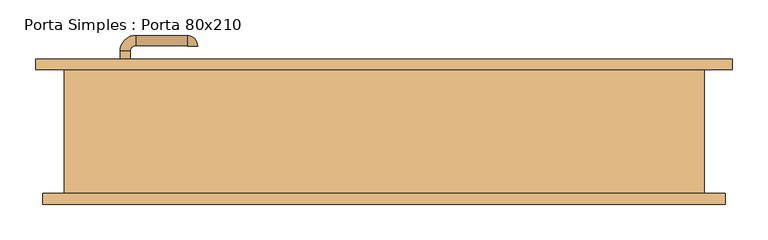
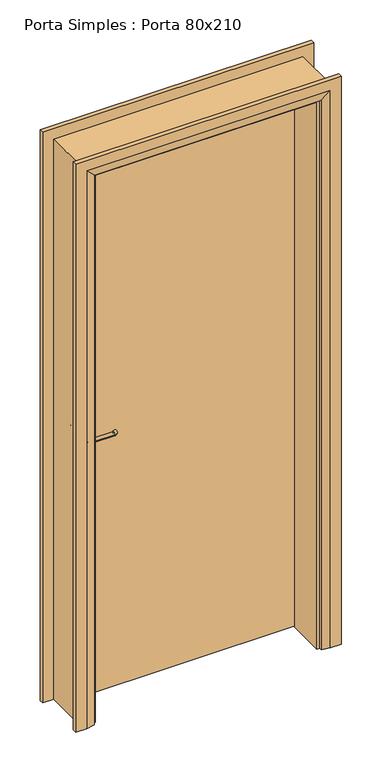
"""IFC4 building model written with IfcOpenShell, lengths in millimetres: door geometry, Porta Simples : Porta 80x210."""

import ifcopenshell
import ifcopenshell.guid

model = None  # the IFC model being written
_history = None  # IfcOwnerHistory: only IFC2X3 demands one
_inside = {}  # id of a spatial element -> (the spatial element, [elements in it])
_under = {}  # id of a project, library or spatial element -> (it, [spatial elements below it])
_declared = {}  # id of a project -> (the project, [libraries it declares])
_typed = {}  # id of a type object -> (the type object, [elements of that type])
_made_of = {}  # id of a material, layer set ... -> (it, [elements and type objects made of it])


def new_model(schema):
    """Start an empty IFC model of exactly this schema.

    Asked for "IFC4X3", IfcOpenShell would pick the latest addendum, in which some entities
    have other attributes; the version numbers below select the first issue.
    IFC2X3 requires an IfcOwnerHistory on every rooted entity: one is made here for all.
    """
    global model, _history
    if schema == "IFC4X3":
        model = ifcopenshell.file(schema_version=(4, 3, 0, 0))
    else:
        model = ifcopenshell.file(schema=schema)
    _inside.clear()
    _under.clear()
    _declared.clear()
    _typed.clear()
    _made_of.clear()
    _history = None
    if model.schema == "IFC2X3":
        org = make("IfcOrganization", Name="unknown")
        user = make(
            "IfcPersonAndOrganization",
            ThePerson=make("IfcPerson", FamilyName="unknown"),
            TheOrganization=org,
        )
        app = make(
            "IfcApplication",
            ApplicationDeveloper=org,
            Version="unknown",
            ApplicationFullName="unknown",
            ApplicationIdentifier="unknown",
        )
        _history = make(
            "IfcOwnerHistory",
            OwningUser=user,
            OwningApplication=app,
            ChangeAction="ADDED",
            CreationDate=0,
        )
    return model


def make(cls, **values):
    """One entity of the class cls with the attributes given. An attribute that is None is left unset."""
    return model.create_entity(
        cls, **{name: value for name, value in values.items() if value is not None}
    )


def rooted(cls, **values):
    """An entity with a GlobalId (a new one), such as an element, a storey or a relation."""
    return make(cls, GlobalId=ifcopenshell.guid.new(), OwnerHistory=_history, **values)


def si_unit(unit_type, name, prefix=None):
    """IfcSIUnit, for example si_unit("LENGTHUNIT", "METRE", prefix="MILLI")."""
    return make("IfcSIUnit", UnitType=unit_type, Prefix=prefix, Name=name)


def assignment(units):
    """IfcUnitAssignment: the units of a project."""
    return None if units is None else make("IfcUnitAssignment", Units=units)


def point(xyz):
    """IfcCartesianPoint."""
    return None if xyz is None else make("IfcCartesianPoint", Coordinates=xyz)


def direction(xyz):
    """IfcDirection."""
    return None if xyz is None else make("IfcDirection", DirectionRatios=xyz)


def frame(location, z_axis=None, x_axis=None):
    """IfcAxis2Placement3D, a coordinate frame: its origin and axes. An axis left out is left unset."""
    return make(
        "IfcAxis2Placement3D",
        Location=point(location),
        Axis=direction(z_axis),
        RefDirection=direction(x_axis),
    )


def frame_2d(location, x_axis=None):
    """IfcAxis2Placement2D, a coordinate frame in the plane: its origin and x axis."""
    return make(
        "IfcAxis2Placement2D", Location=point(location), RefDirection=direction(x_axis)
    )


def origin():
    """The frame at (0, 0, 0) with its axes left unset."""
    return frame((0.0, 0.0, 0.0))


def place(relative_to, where):
    """IfcLocalPlacement: puts the frame where relative to a parent placement (None: the world)."""
    return make(
        "IfcLocalPlacement", PlacementRelTo=relative_to, RelativePlacement=where
    )


def context(
    kind, dimensions, precision=None, world=None, true_north=None, identifier=None
):
    """IfcGeometricRepresentationContext, for example the 3D "Model" context."""
    return make(
        "IfcGeometricRepresentationContext",
        ContextIdentifier=identifier,
        ContextType=kind,
        CoordinateSpaceDimension=dimensions,
        Precision=precision,
        WorldCoordinateSystem=world,
        TrueNorth=true_north,
    )


def project(units=None, contexts=None):
    """IfcProject with its units and contexts."""
    return rooted(
        "IfcProject",
        Name="project",
        RepresentationContexts=contexts,
        UnitsInContext=assignment(units),
    )


def spatial(cls, under=None, at=None, **own):
    """A site, building, storey or space (cls), placed at a placement, below another one or the project."""
    s = rooted(cls, ObjectPlacement=at, **own)
    if under is not None:
        _under.setdefault(under.id(), (under, []))[1].append(s)
    return s


def polyline(points):
    """IfcPolyline through the points."""
    return make("IfcPolyline", Points=[point(p) for p in points])


def circle_curve(where, radius):
    """IfcCircle in the frame where."""
    return make("IfcCircle", Position=where, Radius=radius)


def ellipse_curve(where, semi_axis1, semi_axis2):
    """IfcEllipse in the frame where."""
    return make(
        "IfcEllipse", Position=where, SemiAxis1=semi_axis1, SemiAxis2=semi_axis2
    )


def trimmed(basis, trim1, trim2, sense, master):
    """IfcTrimmedCurve: the piece of a basis curve between two trims."""
    return make(
        "IfcTrimmedCurve",
        BasisCurve=basis,
        Trim1=trim1,
        Trim2=trim2,
        SenseAgreement=sense,
        MasterRepresentation=master,
    )


def segment(curve, same_sense, transition):
    """IfcCompositeCurveSegment."""
    return make(
        "IfcCompositeCurveSegment",
        Transition=transition,
        SameSense=same_sense,
        ParentCurve=curve,
    )


def composite_curve(segments, self_intersect=None):
    """IfcCompositeCurve: segments joined end to end."""
    return make("IfcCompositeCurve", Segments=segments, SelfIntersect=self_intersect)


def outline(outer, holes=None, kind="AREA"):
    """IfcArbitraryClosedProfileDef: a profile drawn as a closed curve; with holes, ...WithVoids."""
    if holes is None:
        return make("IfcArbitraryClosedProfileDef", ProfileType=kind, OuterCurve=outer)
    return make(
        "IfcArbitraryProfileDefWithVoids",
        ProfileType=kind,
        OuterCurve=outer,
        InnerCurves=holes,
    )


def extrude(swept, where, along, depth):
    """IfcExtrudedAreaSolid: the profile swept, set in the frame where, extruded along a direction by depth."""
    return make(
        "IfcExtrudedAreaSolid",
        SweptArea=swept,
        Position=where,
        ExtrudedDirection=direction(along),
        Depth=depth,
    )


def faces_of(points, faces, orient=None, outer=None):
    """IfcFace entities. A face is a list of loops; a loop is a list of indices into points, from 0.

    orient and outer hold one flag for each loop. By default every Orientation is true, the
    first loop of a face is its IfcFaceOuterBound and the others are IfcFaceBound.
    """
    made = []
    for i, loops in enumerate(faces):
        bounds = []
        for j, loop in enumerate(loops):
            is_outer = j == 0 if outer is None else outer[i][j]
            bounds.append(
                make(
                    "IfcFaceOuterBound" if is_outer else "IfcFaceBound",
                    Bound=make("IfcPolyLoop", Polygon=[points[k] for k in loop]),
                    Orientation=True if orient is None else orient[i][j],
                )
            )
        made.append(make("IfcFace", Bounds=bounds))
    return made


def faceted_brep(points, faces, orient=None, outer=None, voids=None):
    """IfcFacetedBrep: a solid bounded by flat faces; with voids (closed shells), ...WithVoids."""
    shared = [point(p) for p in points]
    hull = make("IfcClosedShell", CfsFaces=faces_of(shared, faces, orient, outer))
    if voids is None:
        return make("IfcFacetedBrep", Outer=hull)
    return make(
        "IfcFacetedBrepWithVoids",
        Outer=hull,
        Voids=[
            make(cls, CfsFaces=faces_of(shared, fs, o, b)) for cls, fs, o, b in voids
        ],
    )


def shape(context_of_items, identifier, shape_type, items):
    """IfcShapeRepresentation: the items that make up one representation, for example the "Body"."""
    return make(
        "IfcShapeRepresentation",
        ContextOfItems=context_of_items,
        RepresentationIdentifier=identifier,
        RepresentationType=shape_type,
        Items=items,
    )


def source(mapping_origin, context_of_items, identifier, shape_type, items):
    """IfcRepresentationMap: a shape defined once, which mapped items show again and again."""
    return make(
        "IfcRepresentationMap",
        MappingOrigin=mapping_origin,
        MappedRepresentation=shape(context_of_items, identifier, shape_type, items),
    )


def transform(
    local_origin,
    x_axis=None,
    y_axis=None,
    z_axis=None,
    scale=None,
    scale2=None,
    scale3=None,
    uniform=True,
):
    """IfcCartesianTransformationOperator3D, or its non-uniform kind. x_axis, y_axis, z_axis: its Axis1, 2, 3."""
    if uniform:
        return make(
            "IfcCartesianTransformationOperator3D",
            Axis1=direction(x_axis),
            Axis2=direction(y_axis),
            LocalOrigin=point(local_origin),
            Scale=scale,
            Axis3=direction(z_axis),
        )
    return make(
        "IfcCartesianTransformationOperator3DnonUniform",
        Axis1=direction(x_axis),
        Axis2=direction(y_axis),
        LocalOrigin=point(local_origin),
        Scale=scale,
        Axis3=direction(z_axis),
        Scale2=scale2,
        Scale3=scale3,
    )


def mapped(mapping_source, mapping_target):
    """IfcMappedItem: shows the shape of a source again, moved by a transform."""
    return make(
        "IfcMappedItem", MappingSource=mapping_source, MappingTarget=mapping_target
    )


def made_of(thing, what):
    """Note that an element or type object is made of a material, layer set ...; save() writes the relation."""
    if what is not None:
        _made_of.setdefault(what.id(), (what, []))[1].append(thing)
    return thing


def element(
    cls,
    number,
    at=None,
    inside=None,
    cuts=None,
    type_object=None,
    material=None,
    context=None,
    identifier="Body",
    shape_type=None,
    held_by="IfcProductDefinitionShape",
    body=None,
    shapes=None,
    **own,
):
    """One element of the class cls, such as IfcWall. Its Tag is "e" and its number.

    at: its placement. inside: the storey or other place that contains it. cuts: it is an
    opening in that element (IfcRelVoidsElement). A single representation is given by context,
    identifier, shape_type and body (its items); several are given by shapes. held_by: the class
    of the entity that holds the representations. save() writes the other relations.
    """
    e = rooted(cls, Tag="e%d" % number, ObjectPlacement=at, **own)
    if body is not None:
        shapes = [shape(context, identifier, shape_type, body)]
    if shapes is not None:
        e.Representation = make(held_by, Representations=shapes)
    if inside is not None:
        _inside.setdefault(inside.id(), (inside, []))[1].append(e)
    if cuts is not None:
        rooted(
            "IfcRelVoidsElement", RelatingBuildingElement=cuts, RelatedOpeningElement=e
        )
    if type_object is not None:
        _typed.setdefault(type_object.id(), (type_object, []))[1].append(e)
    return made_of(e, material)


def aggregate(whole, parts):
    """IfcRelAggregates: a whole, such as a stair, and the parts it consists of."""
    return rooted("IfcRelAggregates", RelatingObject=whole, RelatedObjects=parts)


def save(model, path):
    """Write the relations noted so far, then the file.

    IfcRelAggregates (storeys below a building ...), IfcRelContainedInSpatialStructure (elements
    in a storey), IfcRelDefinesByType, IfcRelAssociatesMaterial and IfcRelDeclares: one each for
    every whole, place, type object, material and project.
    """
    for whole, parts in _under.values():
        aggregate(whole, parts)
    for where, things in _inside.values():
        rooted(
            "IfcRelContainedInSpatialStructure",
            RelatedElements=things,
            RelatingStructure=where,
        )
    for kind, things in _typed.values():
        rooted("IfcRelDefinesByType", RelatedObjects=things, RelatingType=kind)
    for what, things in _made_of.values():
        rooted("IfcRelAssociatesMaterial", RelatedObjects=things, RelatingMaterial=what)
    for by, libraries in _declared.values():
        rooted("IfcRelDeclares", RelatingContext=by, RelatedDefinitions=libraries)
    model.write(path)


def plane_surface(at):
    """IfcPlane: the flat surface through the origin of the frame at, square to its z axis."""
    return make("IfcPlane", Position=at)


def cylinder_surface(at, radius):
    """IfcCylindricalSurface: all points at the distance radius from the z axis of the frame at."""
    return make("IfcCylindricalSurface", Position=at, Radius=radius)


def revolved_surface(curve, axis_point, axis_direction):
    """IfcSurfaceOfRevolution: the curve turned about the line through axis_point along axis_direction."""
    return make(
        "IfcSurfaceOfRevolution",
        SweptCurve=make("IfcArbitraryOpenProfileDef", ProfileType="CURVE", Curve=curve),
        AxisPosition=make("IfcAxis1Placement", Location=point(axis_point), Axis=direction(axis_direction)),
    )


def advanced_brep(points, edges, surfaces, faces):
    """IfcAdvancedBrep: a solid bounded by faces that lie on surfaces and meet in shared edges.

    An edge is (start, end): straight between two places in points (the first is 0);
    or (start, end, curve); or (start, end, curve, False) where it runs against its curve.
    A face is (place in surfaces, loops), or (place, loops, False) where it looks against
    its surface's normal. A loop lists edges by number (the first is 1), with a minus sign
    where the edge is run from its end to its start. The first loop is the outer one.
    """
    corners = [point(p) for p in points]
    vertices = [make("IfcVertexPoint", VertexGeometry=c) for c in corners]
    made = []
    for start, end, *more in edges:
        made.append(
            make(
                "IfcEdgeCurve",
                EdgeStart=vertices[start],
                EdgeEnd=vertices[end],
                EdgeGeometry=more[0] if more else make("IfcPolyline", Points=[corners[start], corners[end]]),
                SameSense=more[1] if len(more) > 1 else True,
            )
        )
    hull = []
    for where, loops, *sense in faces:
        bounds = []
        for j, loop in enumerate(loops):
            ring = [make("IfcOrientedEdge", EdgeElement=made[abs(k) - 1], Orientation=k > 0) for k in loop]
            bounds.append(
                make(
                    "IfcFaceOuterBound" if j == 0 else "IfcFaceBound",
                    Bound=make("IfcEdgeLoop", EdgeList=ring),
                    Orientation=True,
                )
            )
        hull.append(make("IfcAdvancedFace", Bounds=bounds, FaceSurface=surfaces[where], SameSense=sense[0] if sense else True))
    return make("IfcAdvancedBrep", Outer=make("IfcClosedShell", CfsFaces=hull))


def porta_simples_porta_80x210_892b00d0(model_context):
    return source(origin(), model_context, "Body", "SolidModel", [
        extrude(outline(composite_curve([segment(trimmed(circle_curve(frame_2d((1050.0, -364.0)), 20.0), [point((1050.0, -384.0))], [point((1050.0, -344.0))], False, "CARTESIAN"), True, "CONTINUOUS"), segment(trimmed(circle_curve(frame_2d((1050.0, -364.0)), 20.0), [point((1050.0, -344.0))], [point((1050.0, -384.0))], False, "CARTESIAN"), True, "CONTINUOUS")], self_intersect=False)), frame((0.0, 41.7070105, 0.0), z_axis=(0.0, 1.0, 0.0), x_axis=(0.0, 0.0, 1.0)), (0.0, 0.0, 1.0), 4.5929895),
        advanced_brep(
        [(-357.0, 41.7070105, 1050.0), (-371.0, 41.7070105, 1050.0), (-371.0, 26.3, 1050.0), (-357.0, 26.3, 1050.0), (-349.0, 4.3, 1050.0), (-349.0, 18.3, 1050.0), (-277.0, 4.3, 1050.0), (-277.0, 18.3, 1050.0), (-276.0, 19.3, 1050.0), (-262.0, 19.3, 1050.0)],
        [
            (0, 1, circle_curve(frame((-364.0, 41.7070105, 1050.0), z_axis=(0.0, 1.0, 0.0), x_axis=(-1.0, 0.0, 0.0)), 7.0)),
            (1, 0, circle_curve(frame((-364.0, 41.7070105, 1050.0), z_axis=(0.0, 1.0, 0.0), x_axis=(-1.0, 0.0, 0.0)), 7.0)),
            (1, 2),
            (2, 3, circle_curve(frame((-364.0, 26.3, 1050.0), z_axis=(0.0, 1.0, 0.0), x_axis=(-1.0, 0.0, 0.0)), 7.0)),
            (3, 0),
            (3, 2, circle_curve(frame((-364.0, 26.3, 1050.0), z_axis=(0.0, 1.0, 0.0), x_axis=(-1.0, 0.0, 0.0)), 7.0)),
            (4, 5, circle_curve(frame((-349.0, 11.3, 1050.0), z_axis=(-1.0, 0.0, 0.0), x_axis=(0.0, -1.0, 0.0)), 7.0)),
            (5, 3, circle_curve(frame((-349.0, 26.3, 1050.0), z_axis=(0.0, 0.0, -1.0), x_axis=(-1.0, 0.0, 0.0)), 8.0)),
            (2, 4, circle_curve(frame((-349.0, 26.3, 1050.0), z_axis=(0.0, 0.0, 1.0), x_axis=(-1.0, 0.0, 0.0)), 22.0)),
            (5, 4, circle_curve(frame((-349.0, 11.3, 1050.0), z_axis=(-1.0, 0.0, 0.0), x_axis=(0.0, -1.0, 0.0)), 7.0)),
            (4, 6),
            (6, 7, circle_curve(frame((-277.0, 11.3, 1050.0), z_axis=(-1.0, 0.0, 0.0), x_axis=(0.0, -1.0, 0.0)), 7.0)),
            (7, 5),
            (7, 6, circle_curve(frame((-277.0, 11.3, 1050.0), z_axis=(-1.0, 0.0, 0.0), x_axis=(0.0, -1.0, 0.0)), 7.0)),
            (8, 9, circle_curve(frame((-269.0, 19.3, 1050.0), z_axis=(0.0, 1.0, 0.0), x_axis=(1.0, 0.0, 0.0)), 7.0)),
            (9, 8, circle_curve(frame((-269.0, 19.3, 1050.0), z_axis=(0.0, 1.0, 0.0), x_axis=(1.0, 0.0, 0.0)), 7.0)),
            (8, 7, circle_curve(frame((-277.0, 19.3, 1050.0), z_axis=(0.0, 0.0, -1.0), x_axis=(0.0, -1.0, 0.0)), 1.0)),
            (6, 9, circle_curve(frame((-277.0, 19.3, 1050.0), z_axis=(0.0, 0.0, 1.0), x_axis=(0.0, -1.0, 0.0)), 15.0)),
        ],
        [
            plane_surface(frame((-364.0, 41.7070105, 1050.0), z_axis=(0.0, 1.0, 0.0), x_axis=(0.0, 0.0, 1.0))),
            cylinder_surface(frame((-364.0, 41.7070105, 1050.0), z_axis=(0.0, 1.0, 0.0), x_axis=(-1.0, 0.0, 0.0)), 7.0),
            revolved_surface(trimmed(ellipse_curve(frame((-364.0, 26.3, 1050.0), z_axis=(0.0, -1.0, 0.0), x_axis=(-1.0, 0.0, 0.0)), 7.0, 7.0), [point((-357.0, 26.3, 1050.0))], [point((-371.0, 26.3, 1050.0))], True, "CARTESIAN"), (-349.0, 26.3, 1050.0), (0.0, 0.0, -1.0)),
            revolved_surface(trimmed(ellipse_curve(frame((-364.0, 26.3, 1050.0), z_axis=(0.0, -1.0, 0.0), x_axis=(-1.0, 0.0, 0.0)), 7.0, 7.0), [point((-371.0, 26.3, 1050.0))], [point((-357.0, 26.3, 1050.0))], True, "CARTESIAN"), (-349.0, 26.3, 1050.0), (0.0, 0.0, -1.0)),
            cylinder_surface(frame((-349.0, 11.3, 1050.0), z_axis=(-1.0, 0.0, 0.0), x_axis=(0.0, -1.0, 0.0)), 7.0),
            plane_surface(frame((-269.0, 19.3, 1050.0), z_axis=(0.0, 1.0, 0.0), x_axis=(0.0, 0.0, 1.0))),
            revolved_surface(trimmed(ellipse_curve(frame((-277.0, 11.3, 1050.0), z_axis=(1.0, 0.0, 0.0), x_axis=(0.0, -1.0, 0.0)), 7.0, 7.0), [point((-277.0, 18.3, 1050.0))], [point((-277.0, 4.3, 1050.0))], True, "CARTESIAN"), (-277.0, 19.3, 1050.0), (0.0, 0.0, -1.0)),
            revolved_surface(trimmed(ellipse_curve(frame((-277.0, 11.3, 1050.0), z_axis=(1.0, 0.0, 0.0), x_axis=(0.0, -1.0, 0.0)), 7.0, 7.0), [point((-277.0, 4.3, 1050.0))], [point((-277.0, 18.3, 1050.0))], True, "CARTESIAN"), (-277.0, 19.3, 1050.0), (0.0, 0.0, -1.0)),
        ],
        [
            (0, [[1, 2]]),
            (1, [[3, 4, 5, -2]]),
            (1, [[-5, 6, -3, -1]]),
            (2, [[7, 8, -4, 9]]),
            (3, [[10, -9, -6, -8]]),
            (4, [[11, 12, 13, -7]]),
            (4, [[-13, 14, -11, -10]]),
            (5, [[15, 16]]),
            (6, [[-15, 17, -12, 18]]),
            (7, [[-16, -18, -14, -17]]),
        ],
    ),
        extrude(outline(polyline([(-334.0, 52.3), (-334.0, 46.3), (-394.0, 46.3), (-394.0, 52.3), (-334.0, 52.3)])), frame((0.0, 0.0, 925.0), z_axis=(0.0, 0.0, 1.0), x_axis=(1.0, 0.0, 0.0)), (0.0, 0.0, 1.0), 165.0),
        extrude(outline(composite_curve([segment(trimmed(circle_curve(frame_2d((1050.0, -364.0)), 20.0), [point((1050.0, -384.0))], [point((1050.0, -344.0))], False, "CARTESIAN"), True, "CONTINUOUS"), segment(trimmed(circle_curve(frame_2d((1050.0, -364.0)), 20.0), [point((1050.0, -344.0))], [point((1050.0, -384.0))], False, "CARTESIAN"), True, "CONTINUOUS")], self_intersect=False)), frame((0.0, 93.3, 0.0), z_axis=(0.0, 1.0, 0.0), x_axis=(0.0, 0.0, 1.0)), (0.0, 0.0, 1.0), 4.5929895),
        advanced_brep(
        [(-357.0, 97.8929895, 1050.0), (-371.0, 97.8929895, 1050.0), (-357.0, 113.3, 1050.0), (-371.0, 113.3, 1050.0), (-349.0, 135.3, 1050.0), (-349.0, 121.3, 1050.0), (-277.0, 121.3, 1050.0), (-277.0, 135.3, 1050.0), (-276.0, 120.3, 1050.0), (-262.0, 120.3, 1050.0)],
        [
            (0, 1, circle_curve(frame((-364.0, 97.8929895, 1050.0), z_axis=(0.0, -1.0, 0.0), x_axis=(-1.0, 0.0, 0.0)), 7.0)),
            (1, 0, circle_curve(frame((-364.0, 97.8929895, 1050.0), z_axis=(0.0, -1.0, 0.0), x_axis=(-1.0, 0.0, 0.0)), 7.0)),
            (0, 2),
            (2, 3, circle_curve(frame((-364.0, 113.3, 1050.0), z_axis=(0.0, -1.0, 0.0), x_axis=(-1.0, 0.0, 0.0)), 7.0)),
            (3, 1),
            (3, 2, circle_curve(frame((-364.0, 113.3, 1050.0), z_axis=(0.0, -1.0, 0.0), x_axis=(-1.0, 0.0, 0.0)), 7.0)),
            (4, 3, circle_curve(frame((-349.0, 113.3, 1050.0), z_axis=(0.0, 0.0, 1.0), x_axis=(-1.0, 0.0, 0.0)), 22.0)),
            (2, 5, circle_curve(frame((-349.0, 113.3, 1050.0), z_axis=(0.0, 0.0, -1.0), x_axis=(-1.0, 0.0, 0.0)), 8.0)),
            (5, 4, circle_curve(frame((-349.0, 128.3, 1050.0), z_axis=(-1.0, 0.0, 0.0), x_axis=(0.0, 1.0, 0.0)), 7.0)),
            (4, 5, circle_curve(frame((-349.0, 128.3, 1050.0), z_axis=(-1.0, 0.0, 0.0), x_axis=(0.0, 1.0, 0.0)), 7.0)),
            (5, 6),
            (6, 7, circle_curve(frame((-277.0, 128.3, 1050.0), z_axis=(-1.0, 0.0, 0.0), x_axis=(0.0, 1.0, 0.0)), 7.0)),
            (7, 4),
            (7, 6, circle_curve(frame((-277.0, 128.3, 1050.0), z_axis=(-1.0, 0.0, 0.0), x_axis=(0.0, 1.0, 0.0)), 7.0)),
            (8, 9, circle_curve(frame((-269.0, 120.3, 1050.0), z_axis=(0.0, -1.0, 0.0), x_axis=(1.0, 0.0, 0.0)), 7.0)),
            (9, 8, circle_curve(frame((-269.0, 120.3, 1050.0), z_axis=(0.0, -1.0, 0.0), x_axis=(1.0, 0.0, 0.0)), 7.0)),
            (9, 7, circle_curve(frame((-277.0, 120.3, 1050.0), z_axis=(0.0, 0.0, 1.0), x_axis=(0.0, 1.0, 0.0)), 15.0)),
            (6, 8, circle_curve(frame((-277.0, 120.3, 1050.0), z_axis=(0.0, 0.0, -1.0), x_axis=(0.0, 1.0, 0.0)), 1.0)),
        ],
        [
            plane_surface(frame((-364.0, 97.8929895, 1050.0), z_axis=(0.0, -1.0, 0.0), x_axis=(0.0, 0.0, 1.0))),
            cylinder_surface(frame((-364.0, 97.8929895, 1050.0), z_axis=(0.0, -1.0, 0.0), x_axis=(-1.0, 0.0, 0.0)), 7.0),
            revolved_surface(trimmed(ellipse_curve(frame((-364.0, 113.3, 1050.0), z_axis=(0.0, -1.0, 0.0), x_axis=(-1.0, 0.0, 0.0)), 7.0, 7.0), [point((-357.0, 113.3, 1050.0))], [point((-371.0, 113.3, 1050.0))], True, "CARTESIAN"), (-349.0, 113.3, 1050.0), (0.0, 0.0, -1.0)),
            revolved_surface(trimmed(ellipse_curve(frame((-364.0, 113.3, 1050.0), z_axis=(0.0, -1.0, 0.0), x_axis=(-1.0, 0.0, 0.0)), 7.0, 7.0), [point((-371.0, 113.3, 1050.0))], [point((-357.0, 113.3, 1050.0))], True, "CARTESIAN"), (-349.0, 113.3, 1050.0), (0.0, 0.0, -1.0)),
            cylinder_surface(frame((-349.0, 128.3, 1050.0), z_axis=(-1.0, 0.0, 0.0), x_axis=(0.0, 1.0, 0.0)), 7.0),
            plane_surface(frame((-269.0, 120.3, 1050.0), z_axis=(0.0, -1.0, 0.0), x_axis=(0.0, 0.0, 1.0))),
            revolved_surface(trimmed(ellipse_curve(frame((-277.0, 128.3, 1050.0), z_axis=(-1.0, 0.0, 0.0), x_axis=(0.0, 1.0, 0.0)), 7.0, 7.0), [point((-277.0, 121.3, 1050.0))], [point((-277.0, 135.3, 1050.0))], True, "CARTESIAN"), (-277.0, 120.3, 1050.0), (0.0, 0.0, -1.0)),
            revolved_surface(trimmed(ellipse_curve(frame((-277.0, 128.3, 1050.0), z_axis=(-1.0, 0.0, 0.0), x_axis=(0.0, 1.0, 0.0)), 7.0, 7.0), [point((-277.0, 135.3, 1050.0))], [point((-277.0, 121.3, 1050.0))], True, "CARTESIAN"), (-277.0, 120.3, 1050.0), (0.0, 0.0, -1.0)),
        ],
        [
            (0, [[1, 2]]),
            (1, [[-1, 3, 4, 5]]),
            (1, [[-2, -5, 6, -3]]),
            (2, [[7, -4, 8, 9]]),
            (3, [[-8, -6, -7, 10]]),
            (4, [[-9, 11, 12, 13]]),
            (4, [[-10, -13, 14, -11]]),
            (5, [[15, 16]]),
            (6, [[17, -12, 18, -16]]),
            (7, [[-18, -14, -17, -15]]),
        ],
    ),
        extrude(outline(polyline([(-334.0, 87.3), (-394.0, 87.3), (-394.0, 93.3), (-334.0, 93.3), (-334.0, 87.3)])), frame((0.0, 0.0, 925.0), z_axis=(0.0, 0.0, 1.0), x_axis=(1.0, 0.0, 0.0)), (0.0, 0.0, 1.0), 165.0),
        extrude(outline(polyline([(408.0, 52.3), (-408.0, 52.3), (-408.0, 87.3), (408.0, 87.3), (408.0, 52.3)])), frame((0.0, 0.0, 53.0), z_axis=(0.0, 0.0, 1.0), x_axis=(1.0, 0.0, 0.0)), (0.0, 0.0, 1.0), 2094.0),
        faceted_brep([(480.0, -87.3, 50.0), (480.0, -102.3, 50.0), (440.0, -102.3, 50.0), (410.0, -97.3, 50.0), (410.0, -87.3, 50.0), (480.0, -87.3, 2220.0), (480.0, -102.3, 2220.0), (-480.0, -102.3, 2220.0), (-480.0, -102.3, 50.0), (-440.0, -102.3, 50.0), (-440.0, -102.3, 2180.0), (440.0, -102.3, 2180.0), (410.0, -97.3, 2150.0), (410.0, -87.3, 2150.0), (-410.0, -87.3, 2150.0), (-410.0, -87.3, 50.0), (-480.0, -87.3, 50.0), (-480.0, -87.3, 2220.0), (-410.0, -97.3, 2150.0), (-410.0, -97.3, 50.0)], [[[0, 1, 2, 3, 4]], [[1, 0, 5, 6]], [[2, 1, 6, 7, 8, 9, 10, 11]], [[3, 2, 11, 12]], [[4, 3, 12, 13]], [[0, 4, 13, 14, 15, 16, 17, 5]], [[14, 18, 19, 15]], [[16, 15, 19, 9, 8]], [[7, 17, 16, 8]], [[18, 10, 9, 19]], [[13, 12, 18, 14]], [[6, 5, 17, 7]], [[12, 11, 10, 18]]]),
        faceted_brep([(490.0, 87.3, 50.0), (420.0, 87.3, 50.0), (420.0, 97.3, 50.0), (450.0, 102.3, 50.0), (490.0, 102.3, 50.0), (490.0, 87.3, 2230.0), (-490.0, 87.3, 2230.0), (-490.0, 87.3, 50.0), (-420.0, 87.3, 50.0), (-420.0, 87.3, 2160.0), (420.0, 87.3, 2160.0), (420.0, 97.3, 2160.0), (450.0, 102.3, 2190.0), (-450.0, 102.3, 2190.0), (-450.0, 102.3, 50.0), (-490.0, 102.3, 50.0), (-490.0, 102.3, 2230.0), (490.0, 102.3, 2230.0), (-420.0, 97.3, 50.0), (-420.0, 97.3, 2160.0)], [[[0, 1, 2, 3, 4]], [[1, 0, 5, 6, 7, 8, 9, 10]], [[2, 1, 10, 11]], [[3, 2, 11, 12]], [[4, 3, 12, 13, 14, 15, 16, 17]], [[0, 4, 17, 5]], [[6, 16, 15, 7]], [[7, 15, 14, 18, 8]], [[19, 9, 8, 18]], [[13, 19, 18, 14]], [[11, 10, 9, 19]], [[5, 17, 16, 6]], [[12, 11, 19, 13]]]),
        faceted_brep([(-410.0, 87.3, 50.0), (-410.0, 50.3, 50.0), (-400.0, 50.3, 50.0), (-400.0, -87.3, 50.0), (-450.0, -87.3, 50.0), (-450.0, 87.3, 50.0), (-410.0, 87.3, 2150.0), (-410.0, 50.3, 2150.0), (-400.0, 50.3, 2140.0), (-400.0, -87.3, 2140.0), (-450.0, -87.3, 2190.0), (-450.0, 87.3, 2190.0), (410.0, 87.3, 50.0), (450.0, 87.3, 50.0), (450.0, -87.3, 50.0), (400.0, -87.3, 50.0), (400.0, 50.3, 50.0), (410.0, 50.3, 50.0), (410.0, 87.3, 2150.0), (450.0, 87.3, 2190.0), (450.0, -87.3, 2190.0), (400.0, -87.3, 2140.0), (400.0, 50.3, 2140.0), (410.0, 50.3, 2150.0)], [[[0, 1, 2, 3, 4, 5]], [[1, 0, 6, 7]], [[2, 1, 7, 8]], [[3, 2, 8, 9]], [[4, 3, 9, 10]], [[5, 4, 10, 11]], [[0, 5, 11, 6]], [[12, 13, 14, 15, 16, 17]], [[18, 19, 13, 12]], [[19, 20, 14, 13]], [[20, 21, 15, 14]], [[21, 22, 16, 15]], [[22, 23, 17, 16]], [[23, 18, 12, 17]], [[7, 6, 18, 23]], [[8, 7, 23, 22]], [[9, 8, 22, 21]], [[10, 9, 21, 20]], [[11, 10, 20, 19]], [[6, 11, 19, 18]]]),
    ])


if __name__ == "__main__":
    model = new_model("IFC4")
    model_context = context("Model", 3, world=origin())
    ifc_project = project(units=[si_unit("LENGTHUNIT", "METRE", prefix="MILLI")], contexts=[model_context])
    site = spatial("IfcSite", under=ifc_project)
    building = spatial("IfcBuilding", under=site)
    placement = place(None, origin())
    porta_simples_porta_80x210_shape = porta_simples_porta_80x210_892b00d0(model_context)
    element("IfcDoor", 1, ObjectType="Porta Simples : Porta 80x210", at=placement, inside=building, context=model_context, shape_type="MappedRepresentation", body=[
        mapped(porta_simples_porta_80x210_shape, transform((0.0, 0.0, 0.0), x_axis=(1.0, 0.0, 0.0), y_axis=(0.0, 1.0, 0.0), z_axis=(0.0, 0.0, 1.0))),
    ])
    save(model, "model.ifc")

# Revit data of these elements
# Type "Porta Simples : Porta 80x210"
#   Type Mark = "49"
#   SINAPI = ""
#   Analytic Construction = "<Nenhum>"
#   Construction Type = "300"
#   Maçaneta [instance default] = ""
#   Fechadura [instance default] = ""
#   Vão Luz (somente para informação) = 0.78 m
#   Tolerância Folha Vertical = 0.003 m
#   Módulo Básico M = 0.10 m
#   Largura de Coordenação Modular Largura CM = 0.90 m
#   Rough Width = 0.90 m
#   Deslocamento da Horizontal da Folha = 0.00 m
#   Altura de Coordenação Modular Largura CM = 2.20 m
#   Rough Height = 2.20 m
#   Altura Nominal = 2.09 m
#   Ajuste de Coordenação Topo AC Topo = 0.01 m
#   Ajuste de Coordenação Base AC Base = 0.05 m
#   Ajuste de Coordenação AC = 0.01 m
#   Tolerância Folha Horizontal = 0.002 m
#   Largura Folha (somente para informação) = 0.796 m
#   Espessura Folha = 0.035 m
#   Maçaneta - Distância da Folha = 0.044 m
#   Maçaneta - Altura = 1.00 m
#   Largura Nominal (Largura Mn) = 0.82 m
#   Distância do Nível = 0.003 m
#   Aduela Interna Espessura = 0.04 m
#   Aduela Externa Espessura = 0.05 m
#   Altura Folha (somente para informação) = 2.075 m
#   Height = 2.14 m
#   Width = 0.88 m
#   Número de Módulos Básicos nM Largura = 9
#   Número de Módulos Básicos nM Altura = 22
#   Marco Metálico = no
#   Aduela de Madeira = no
#   Aduela Metálica de Canto = no
#   Guarnição Reta = no
#   Guarnição Chanfrada = yes
#   Batente - Material [instance default] = none
#   Painel - Material [instance default] = none
#   Model = ""
#   Function = (empty or 0)
#   Description = (empty or 0)
#   Wall Closure = (empty or 0)
#   Assembly Code = ""
# Element 1 (IfcDoor, "Porta Simples : Porta 80x210")
#   Materials on its faces: "Porta - Maçaneta"
# Materials
#   "Porta - Maçaneta": class "Diversos", colour RGB 0 0 0, transparency 0
